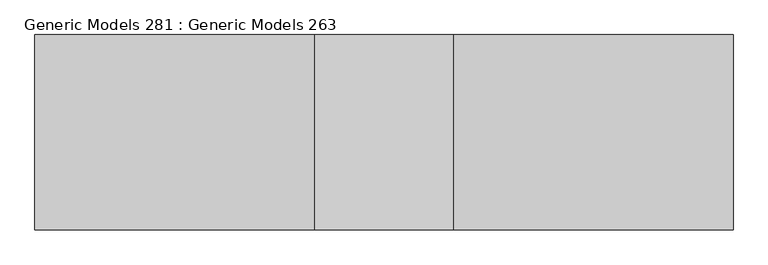
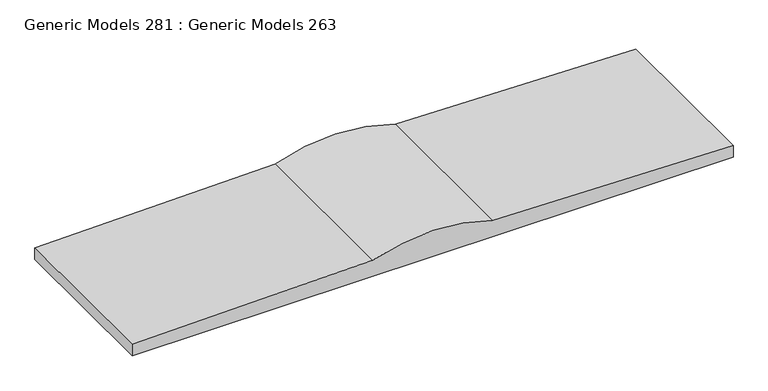
"""IFC4 building model written with IfcOpenShell, lengths in millimetres: proxy geometry, Generic Models 281 : Generic Models 263."""

import ifcopenshell
import ifcopenshell.guid

model = None  # the IFC model being written
_history = None  # IfcOwnerHistory: only IFC2X3 demands one
_inside = {}  # id of a spatial element -> (the spatial element, [elements in it])
_under = {}  # id of a project, library or spatial element -> (it, [spatial elements below it])
_declared = {}  # id of a project -> (the project, [libraries it declares])
_typed = {}  # id of a type object -> (the type object, [elements of that type])
_made_of = {}  # id of a material, layer set ... -> (it, [elements and type objects made of it])


def new_model(schema):
    """Start an empty IFC model of exactly this schema.

    Asked for "IFC4X3", IfcOpenShell would pick the latest addendum, in which some entities
    have other attributes; the version numbers below select the first issue.
    IFC2X3 requires an IfcOwnerHistory on every rooted entity: one is made here for all.
    """
    global model, _history
    if schema == "IFC4X3":
        model = ifcopenshell.file(schema_version=(4, 3, 0, 0))
    else:
        model = ifcopenshell.file(schema=schema)
    _inside.clear()
    _under.clear()
    _declared.clear()
    _typed.clear()
    _made_of.clear()
    _history = None
    if model.schema == "IFC2X3":
        org = make("IfcOrganization", Name="unknown")
        user = make(
            "IfcPersonAndOrganization",
            ThePerson=make("IfcPerson", FamilyName="unknown"),
            TheOrganization=org,
        )
        app = make(
            "IfcApplication",
            ApplicationDeveloper=org,
            Version="unknown",
            ApplicationFullName="unknown",
            ApplicationIdentifier="unknown",
        )
        _history = make(
            "IfcOwnerHistory",
            OwningUser=user,
            OwningApplication=app,
            ChangeAction="ADDED",
            CreationDate=0,
        )
    return model


def make(cls, **values):
    """One entity of the class cls with the attributes given. An attribute that is None is left unset."""
    return model.create_entity(
        cls, **{name: value for name, value in values.items() if value is not None}
    )


def rooted(cls, **values):
    """An entity with a GlobalId (a new one), such as an element, a storey or a relation."""
    return make(cls, GlobalId=ifcopenshell.guid.new(), OwnerHistory=_history, **values)


def si_unit(unit_type, name, prefix=None):
    """IfcSIUnit, for example si_unit("LENGTHUNIT", "METRE", prefix="MILLI")."""
    return make("IfcSIUnit", UnitType=unit_type, Prefix=prefix, Name=name)


def assignment(units):
    """IfcUnitAssignment: the units of a project."""
    return None if units is None else make("IfcUnitAssignment", Units=units)


def point(xyz):
    """IfcCartesianPoint."""
    return None if xyz is None else make("IfcCartesianPoint", Coordinates=xyz)


def direction(xyz):
    """IfcDirection."""
    return None if xyz is None else make("IfcDirection", DirectionRatios=xyz)


def frame(location, z_axis=None, x_axis=None):
    """IfcAxis2Placement3D, a coordinate frame: its origin and axes. An axis left out is left unset."""
    return make(
        "IfcAxis2Placement3D",
        Location=point(location),
        Axis=direction(z_axis),
        RefDirection=direction(x_axis),
    )


def frame_2d(location, x_axis=None):
    """IfcAxis2Placement2D, a coordinate frame in the plane: its origin and x axis."""
    return make(
        "IfcAxis2Placement2D", Location=point(location), RefDirection=direction(x_axis)
    )


def origin():
    """The frame at (0, 0, 0) with its axes left unset."""
    return frame((0.0, 0.0, 0.0))


def place(relative_to, where):
    """IfcLocalPlacement: puts the frame where relative to a parent placement (None: the world)."""
    return make(
        "IfcLocalPlacement", PlacementRelTo=relative_to, RelativePlacement=where
    )


def context(
    kind, dimensions, precision=None, world=None, true_north=None, identifier=None
):
    """IfcGeometricRepresentationContext, for example the 3D "Model" context."""
    return make(
        "IfcGeometricRepresentationContext",
        ContextIdentifier=identifier,
        ContextType=kind,
        CoordinateSpaceDimension=dimensions,
        Precision=precision,
        WorldCoordinateSystem=world,
        TrueNorth=true_north,
    )


def project(units=None, contexts=None):
    """IfcProject with its units and contexts."""
    return rooted(
        "IfcProject",
        Name="project",
        RepresentationContexts=contexts,
        UnitsInContext=assignment(units),
    )


def spatial(cls, under=None, at=None, **own):
    """A site, building, storey or space (cls), placed at a placement, below another one or the project."""
    s = rooted(cls, ObjectPlacement=at, **own)
    if under is not None:
        _under.setdefault(under.id(), (under, []))[1].append(s)
    return s


def polyline(points):
    """IfcPolyline through the points."""
    return make("IfcPolyline", Points=[point(p) for p in points])


def circle_curve(where, radius):
    """IfcCircle in the frame where."""
    return make("IfcCircle", Position=where, Radius=radius)


def trimmed(basis, trim1, trim2, sense, master):
    """IfcTrimmedCurve: the piece of a basis curve between two trims."""
    return make(
        "IfcTrimmedCurve",
        BasisCurve=basis,
        Trim1=trim1,
        Trim2=trim2,
        SenseAgreement=sense,
        MasterRepresentation=master,
    )


def segment(curve, same_sense, transition):
    """IfcCompositeCurveSegment."""
    return make(
        "IfcCompositeCurveSegment",
        Transition=transition,
        SameSense=same_sense,
        ParentCurve=curve,
    )


def composite_curve(segments, self_intersect=None):
    """IfcCompositeCurve: segments joined end to end."""
    return make("IfcCompositeCurve", Segments=segments, SelfIntersect=self_intersect)


def outline(outer, holes=None, kind="AREA"):
    """IfcArbitraryClosedProfileDef: a profile drawn as a closed curve; with holes, ...WithVoids."""
    if holes is None:
        return make("IfcArbitraryClosedProfileDef", ProfileType=kind, OuterCurve=outer)
    return make(
        "IfcArbitraryProfileDefWithVoids",
        ProfileType=kind,
        OuterCurve=outer,
        InnerCurves=holes,
    )


def extrude(swept, where, along, depth):
    """IfcExtrudedAreaSolid: the profile swept, set in the frame where, extruded along a direction by depth."""
    return make(
        "IfcExtrudedAreaSolid",
        SweptArea=swept,
        Position=where,
        ExtrudedDirection=direction(along),
        Depth=depth,
    )


def shape(context_of_items, identifier, shape_type, items):
    """IfcShapeRepresentation: the items that make up one representation, for example the "Body"."""
    return make(
        "IfcShapeRepresentation",
        ContextOfItems=context_of_items,
        RepresentationIdentifier=identifier,
        RepresentationType=shape_type,
        Items=items,
    )


def source(mapping_origin, context_of_items, identifier, shape_type, items):
    """IfcRepresentationMap: a shape defined once, which mapped items show again and again."""
    return make(
        "IfcRepresentationMap",
        MappingOrigin=mapping_origin,
        MappedRepresentation=shape(context_of_items, identifier, shape_type, items),
    )


def transform(
    local_origin,
    x_axis=None,
    y_axis=None,
    z_axis=None,
    scale=None,
    scale2=None,
    scale3=None,
    uniform=True,
):
    """IfcCartesianTransformationOperator3D, or its non-uniform kind. x_axis, y_axis, z_axis: its Axis1, 2, 3."""
    if uniform:
        return make(
            "IfcCartesianTransformationOperator3D",
            Axis1=direction(x_axis),
            Axis2=direction(y_axis),
            LocalOrigin=point(local_origin),
            Scale=scale,
            Axis3=direction(z_axis),
        )
    return make(
        "IfcCartesianTransformationOperator3DnonUniform",
        Axis1=direction(x_axis),
        Axis2=direction(y_axis),
        LocalOrigin=point(local_origin),
        Scale=scale,
        Axis3=direction(z_axis),
        Scale2=scale2,
        Scale3=scale3,
    )


def mapped(mapping_source, mapping_target):
    """IfcMappedItem: shows the shape of a source again, moved by a transform."""
    return make(
        "IfcMappedItem", MappingSource=mapping_source, MappingTarget=mapping_target
    )


def made_of(thing, what):
    """Note that an element or type object is made of a material, layer set ...; save() writes the relation."""
    if what is not None:
        _made_of.setdefault(what.id(), (what, []))[1].append(thing)
    return thing


def element(
    cls,
    number,
    at=None,
    inside=None,
    cuts=None,
    type_object=None,
    material=None,
    context=None,
    identifier="Body",
    shape_type=None,
    held_by="IfcProductDefinitionShape",
    body=None,
    shapes=None,
    **own,
):
    """One element of the class cls, such as IfcWall. Its Tag is "e" and its number.

    at: its placement. inside: the storey or other place that contains it. cuts: it is an
    opening in that element (IfcRelVoidsElement). A single representation is given by context,
    identifier, shape_type and body (its items); several are given by shapes. held_by: the class
    of the entity that holds the representations. save() writes the other relations.
    """
    e = rooted(cls, Tag="e%d" % number, ObjectPlacement=at, **own)
    if body is not None:
        shapes = [shape(context, identifier, shape_type, body)]
    if shapes is not None:
        e.Representation = make(held_by, Representations=shapes)
    if inside is not None:
        _inside.setdefault(inside.id(), (inside, []))[1].append(e)
    if cuts is not None:
        rooted(
            "IfcRelVoidsElement", RelatingBuildingElement=cuts, RelatedOpeningElement=e
        )
    if type_object is not None:
        _typed.setdefault(type_object.id(), (type_object, []))[1].append(e)
    return made_of(e, material)


def aggregate(whole, parts):
    """IfcRelAggregates: a whole, such as a stair, and the parts it consists of."""
    return rooted("IfcRelAggregates", RelatingObject=whole, RelatedObjects=parts)


def save(model, path):
    """Write the relations noted so far, then the file.

    IfcRelAggregates (storeys below a building ...), IfcRelContainedInSpatialStructure (elements
    in a storey), IfcRelDefinesByType, IfcRelAssociatesMaterial and IfcRelDeclares: one each for
    every whole, place, type object, material and project.
    """
    for whole, parts in _under.values():
        aggregate(whole, parts)
    for where, things in _inside.values():
        rooted(
            "IfcRelContainedInSpatialStructure",
            RelatedElements=things,
            RelatingStructure=where,
        )
    for kind, things in _typed.values():
        rooted("IfcRelDefinesByType", RelatedObjects=things, RelatingType=kind)
    for what, things in _made_of.values():
        rooted("IfcRelAssociatesMaterial", RelatedObjects=things, RelatingMaterial=what)
    for by, libraries in _declared.values():
        rooted("IfcRelDeclares", RelatingContext=by, RelatedDefinitions=libraries)
    model.write(path)


def generic_models_281_generic_models_263_cbb34a41(model_context):
    return source(origin(), model_context, "Body", "SweptSolid", [
        extrude(outline(composite_curve([segment(polyline([(0.0, 64122.5797726), (-304.9836851, 64122.5797726)]), True, "CONTINUOUS"), segment(trimmed(circle_curve(frame_2d((-219607.3320282, 71742.5797726)), 219434.6927648), [point((-304.9836851, 64122.5797726))], [point((-304.9836851, 79362.5797726))], True, "CARTESIAN"), True, "CONTINUOUS"), segment(polyline([(-304.9836851, 79362.5797726), (0.0, 79362.5797726)]), True, "CONTINUOUS"), segment(trimmed(circle_curve(frame_2d((-219607.3320282, 71742.5797726)), 219739.4927648), [point((0.0, 79362.5797726))], [point((126.8758334, 73266.5797726))], False, "CARTESIAN"), True, "CONTINUOUS"), segment(trimmed(circle_curve(frame_2d((-4163.1944851, 71742.5797726)), 4552.7221898), [point((126.8758334, 73266.5797726))], [point((126.8758334, 70218.5797726))], False, "CARTESIAN"), True, "CONTINUOUS"), segment(trimmed(circle_curve(frame_2d((-219607.3320282, 71742.5797726)), 219739.4927648), [point((126.8758334, 70218.5797726))], [point((0.0, 64122.5797726))], False, "CARTESIAN"), True, "CONTINUOUS")], self_intersect=False)), frame((0.0, -1618.4486541, 0.0), z_axis=(0.0, 1.0, 0.0), x_axis=(0.0, 0.0, 1.0)), (0.0, 0.0, 1.0), 4267.2),
    ])


if __name__ == "__main__":
    model = new_model("IFC4")
    model_context = context("Model", 3, world=origin())
    ifc_project = project(units=[si_unit("LENGTHUNIT", "METRE", prefix="MILLI")], contexts=[model_context])
    site = spatial("IfcSite", under=ifc_project)
    building = spatial("IfcBuilding", under=site)
    placement = place(None, origin())
    generic_models_281_generic_models_263_shape = generic_models_281_generic_models_263_cbb34a41(model_context)
    element("IfcBuildingElementProxy", 1, Name="Generic Models 281 : Generic Models 263", ObjectType="Generic Models 281 : Generic Models 263", at=placement, inside=building, context=model_context, shape_type="MappedRepresentation", body=[
        mapped(generic_models_281_generic_models_263_shape, transform((0.0, 0.0, 0.0), x_axis=(1.0, 0.0, 0.0), y_axis=(0.0, 1.0, 0.0), z_axis=(0.0, 0.0, 1.0))),
    ])
    save(model, "model.ifc")

# Revit data of these elements
# Element 1 (IfcBuildingElementProxy, "Generic Models 281 : Generic Models 263")
#   Materials on its faces: "3\" TO 6\" WASHED OR CLEAR STONE"
# Materials
#   "3\" TO 6\" WASHED OR CLEAR STONE": class "Miscellaneous", colour RGB 210 210 210, transparency 0, Cost = 0
